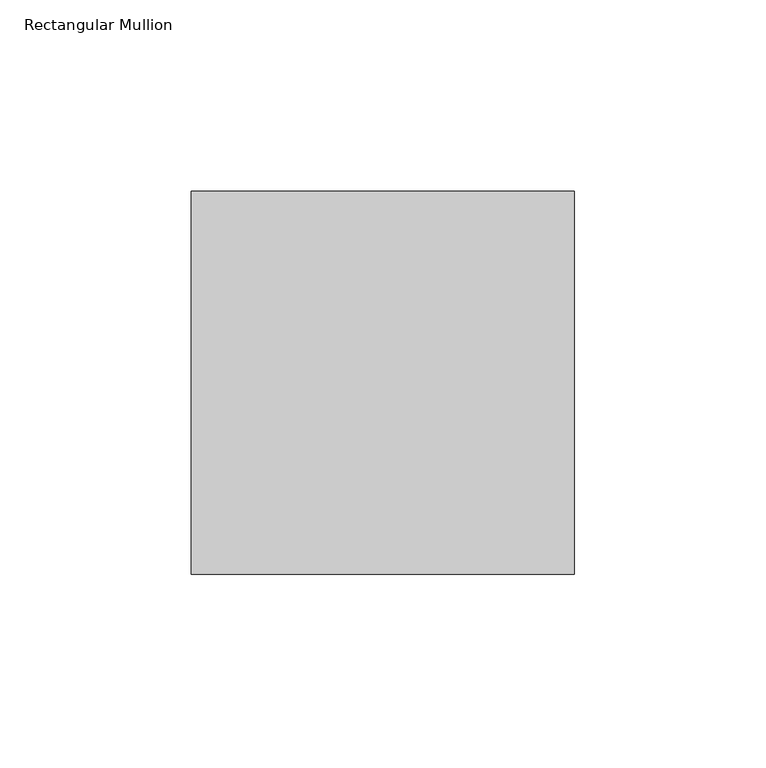
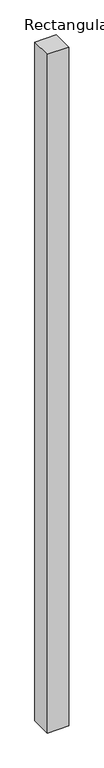
"""IFC4 building model written with IfcOpenShell, lengths in millimetres: member geometry, Rectangular Mullion : 알루미늄_Rectangular Cap_100 x100."""

import ifcopenshell
import ifcopenshell.guid

model = None  # the IFC model being written
_history = None  # IfcOwnerHistory: only IFC2X3 demands one
_inside = {}  # id of a spatial element -> (the spatial element, [elements in it])
_under = {}  # id of a project, library or spatial element -> (it, [spatial elements below it])
_declared = {}  # id of a project -> (the project, [libraries it declares])
_typed = {}  # id of a type object -> (the type object, [elements of that type])
_made_of = {}  # id of a material, layer set ... -> (it, [elements and type objects made of it])


def new_model(schema):
    """Start an empty IFC model of exactly this schema.

    Asked for "IFC4X3", IfcOpenShell would pick the latest addendum, in which some entities
    have other attributes; the version numbers below select the first issue.
    IFC2X3 requires an IfcOwnerHistory on every rooted entity: one is made here for all.
    """
    global model, _history
    if schema == "IFC4X3":
        model = ifcopenshell.file(schema_version=(4, 3, 0, 0))
    else:
        model = ifcopenshell.file(schema=schema)
    _inside.clear()
    _under.clear()
    _declared.clear()
    _typed.clear()
    _made_of.clear()
    _history = None
    if model.schema == "IFC2X3":
        org = make("IfcOrganization", Name="unknown")
        user = make(
            "IfcPersonAndOrganization",
            ThePerson=make("IfcPerson", FamilyName="unknown"),
            TheOrganization=org,
        )
        app = make(
            "IfcApplication",
            ApplicationDeveloper=org,
            Version="unknown",
            ApplicationFullName="unknown",
            ApplicationIdentifier="unknown",
        )
        _history = make(
            "IfcOwnerHistory",
            OwningUser=user,
            OwningApplication=app,
            ChangeAction="ADDED",
            CreationDate=0,
        )
    return model


def make(cls, **values):
    """One entity of the class cls with the attributes given. An attribute that is None is left unset."""
    return model.create_entity(
        cls, **{name: value for name, value in values.items() if value is not None}
    )


def rooted(cls, **values):
    """An entity with a GlobalId (a new one), such as an element, a storey or a relation."""
    return make(cls, GlobalId=ifcopenshell.guid.new(), OwnerHistory=_history, **values)


def si_unit(unit_type, name, prefix=None):
    """IfcSIUnit, for example si_unit("LENGTHUNIT", "METRE", prefix="MILLI")."""
    return make("IfcSIUnit", UnitType=unit_type, Prefix=prefix, Name=name)


def assignment(units):
    """IfcUnitAssignment: the units of a project."""
    return None if units is None else make("IfcUnitAssignment", Units=units)


def point(xyz):
    """IfcCartesianPoint."""
    return None if xyz is None else make("IfcCartesianPoint", Coordinates=xyz)


def direction(xyz):
    """IfcDirection."""
    return None if xyz is None else make("IfcDirection", DirectionRatios=xyz)


def frame(location, z_axis=None, x_axis=None):
    """IfcAxis2Placement3D, a coordinate frame: its origin and axes. An axis left out is left unset."""
    return make(
        "IfcAxis2Placement3D",
        Location=point(location),
        Axis=direction(z_axis),
        RefDirection=direction(x_axis),
    )


def origin():
    """The frame at (0, 0, 0) with its axes left unset."""
    return frame((0.0, 0.0, 0.0))


def place(relative_to, where):
    """IfcLocalPlacement: puts the frame where relative to a parent placement (None: the world)."""
    return make(
        "IfcLocalPlacement", PlacementRelTo=relative_to, RelativePlacement=where
    )


def context(
    kind, dimensions, precision=None, world=None, true_north=None, identifier=None
):
    """IfcGeometricRepresentationContext, for example the 3D "Model" context."""
    return make(
        "IfcGeometricRepresentationContext",
        ContextIdentifier=identifier,
        ContextType=kind,
        CoordinateSpaceDimension=dimensions,
        Precision=precision,
        WorldCoordinateSystem=world,
        TrueNorth=true_north,
    )


def project(units=None, contexts=None):
    """IfcProject with its units and contexts."""
    return rooted(
        "IfcProject",
        Name="project",
        RepresentationContexts=contexts,
        UnitsInContext=assignment(units),
    )


def spatial(cls, under=None, at=None, **own):
    """A site, building, storey or space (cls), placed at a placement, below another one or the project."""
    s = rooted(cls, ObjectPlacement=at, **own)
    if under is not None:
        _under.setdefault(under.id(), (under, []))[1].append(s)
    return s


def polyline(points):
    """IfcPolyline through the points."""
    return make("IfcPolyline", Points=[point(p) for p in points])


def outline(outer, holes=None, kind="AREA"):
    """IfcArbitraryClosedProfileDef: a profile drawn as a closed curve; with holes, ...WithVoids."""
    if holes is None:
        return make("IfcArbitraryClosedProfileDef", ProfileType=kind, OuterCurve=outer)
    return make(
        "IfcArbitraryProfileDefWithVoids",
        ProfileType=kind,
        OuterCurve=outer,
        InnerCurves=holes,
    )


def extrude(swept, where, along, depth):
    """IfcExtrudedAreaSolid: the profile swept, set in the frame where, extruded along a direction by depth."""
    return make(
        "IfcExtrudedAreaSolid",
        SweptArea=swept,
        Position=where,
        ExtrudedDirection=direction(along),
        Depth=depth,
    )


def shape(context_of_items, identifier, shape_type, items):
    """IfcShapeRepresentation: the items that make up one representation, for example the "Body"."""
    return make(
        "IfcShapeRepresentation",
        ContextOfItems=context_of_items,
        RepresentationIdentifier=identifier,
        RepresentationType=shape_type,
        Items=items,
    )


def source(mapping_origin, context_of_items, identifier, shape_type, items):
    """IfcRepresentationMap: a shape defined once, which mapped items show again and again."""
    return make(
        "IfcRepresentationMap",
        MappingOrigin=mapping_origin,
        MappedRepresentation=shape(context_of_items, identifier, shape_type, items),
    )


def transform(
    local_origin,
    x_axis=None,
    y_axis=None,
    z_axis=None,
    scale=None,
    scale2=None,
    scale3=None,
    uniform=True,
):
    """IfcCartesianTransformationOperator3D, or its non-uniform kind. x_axis, y_axis, z_axis: its Axis1, 2, 3."""
    if uniform:
        return make(
            "IfcCartesianTransformationOperator3D",
            Axis1=direction(x_axis),
            Axis2=direction(y_axis),
            LocalOrigin=point(local_origin),
            Scale=scale,
            Axis3=direction(z_axis),
        )
    return make(
        "IfcCartesianTransformationOperator3DnonUniform",
        Axis1=direction(x_axis),
        Axis2=direction(y_axis),
        LocalOrigin=point(local_origin),
        Scale=scale,
        Axis3=direction(z_axis),
        Scale2=scale2,
        Scale3=scale3,
    )


def mapped(mapping_source, mapping_target):
    """IfcMappedItem: shows the shape of a source again, moved by a transform."""
    return make(
        "IfcMappedItem", MappingSource=mapping_source, MappingTarget=mapping_target
    )


def made_of(thing, what):
    """Note that an element or type object is made of a material, layer set ...; save() writes the relation."""
    if what is not None:
        _made_of.setdefault(what.id(), (what, []))[1].append(thing)
    return thing


def element(
    cls,
    number,
    at=None,
    inside=None,
    cuts=None,
    type_object=None,
    material=None,
    context=None,
    identifier="Body",
    shape_type=None,
    held_by="IfcProductDefinitionShape",
    body=None,
    shapes=None,
    **own,
):
    """One element of the class cls, such as IfcWall. Its Tag is "e" and its number.

    at: its placement. inside: the storey or other place that contains it. cuts: it is an
    opening in that element (IfcRelVoidsElement). A single representation is given by context,
    identifier, shape_type and body (its items); several are given by shapes. held_by: the class
    of the entity that holds the representations. save() writes the other relations.
    """
    e = rooted(cls, Tag="e%d" % number, ObjectPlacement=at, **own)
    if body is not None:
        shapes = [shape(context, identifier, shape_type, body)]
    if shapes is not None:
        e.Representation = make(held_by, Representations=shapes)
    if inside is not None:
        _inside.setdefault(inside.id(), (inside, []))[1].append(e)
    if cuts is not None:
        rooted(
            "IfcRelVoidsElement", RelatingBuildingElement=cuts, RelatedOpeningElement=e
        )
    if type_object is not None:
        _typed.setdefault(type_object.id(), (type_object, []))[1].append(e)
    return made_of(e, material)


def aggregate(whole, parts):
    """IfcRelAggregates: a whole, such as a stair, and the parts it consists of."""
    return rooted("IfcRelAggregates", RelatingObject=whole, RelatedObjects=parts)


def save(model, path):
    """Write the relations noted so far, then the file.

    IfcRelAggregates (storeys below a building ...), IfcRelContainedInSpatialStructure (elements
    in a storey), IfcRelDefinesByType, IfcRelAssociatesMaterial and IfcRelDeclares: one each for
    every whole, place, type object, material and project.
    """
    for whole, parts in _under.values():
        aggregate(whole, parts)
    for where, things in _inside.values():
        rooted(
            "IfcRelContainedInSpatialStructure",
            RelatedElements=things,
            RelatingStructure=where,
        )
    for kind, things in _typed.values():
        rooted("IfcRelDefinesByType", RelatedObjects=things, RelatingType=kind)
    for what, things in _made_of.values():
        rooted("IfcRelAssociatesMaterial", RelatedObjects=things, RelatingMaterial=what)
    for by, libraries in _declared.values():
        rooted("IfcRelDeclares", RelatingContext=by, RelatedDefinitions=libraries)
    model.write(path)


def rectangular_mullion_9dbe7c8d(model_context):
    return source(origin(), model_context, "Body", "SweptSolid", [
        extrude(outline(polyline([(0.0, 50.0), (0.0, -50.0), (-100.0, -50.0), (-100.0, 50.0), (0.0, 50.0)])), frame((0.0, 0.0, -3325.0), z_axis=(0.0, 0.0, 1.0), x_axis=(1.0, 0.0, 0.0)), (0.0, 0.0, 1.0), 3325.0),
    ])


if __name__ == "__main__":
    model = new_model("IFC4")
    model_context = context("Model", 3, world=origin())
    ifc_project = project(units=[si_unit("LENGTHUNIT", "METRE", prefix="MILLI")], contexts=[model_context])
    site = spatial("IfcSite", under=ifc_project)
    building = spatial("IfcBuilding", under=site)
    placement = place(None, origin())
    rectangular_mullion_shape = rectangular_mullion_9dbe7c8d(model_context)
    element("IfcMember", 1, ObjectType="Rectangular Mullion : 알루미늄_Rectangular Cap_100 x100", at=placement, inside=building, context=model_context, shape_type="MappedRepresentation", body=[
        mapped(rectangular_mullion_shape, transform((0.0, 0.0, 0.0), x_axis=(1.0, 0.0, 0.0), y_axis=(0.0, 1.0, 0.0), z_axis=(0.0, 0.0, 1.0))),
    ])
    save(model, "model.ifc")

# Revit data of these elements
# Type "Rectangular Mullion : 알루미늄_Rectangular Cap_100 x100"
#   built-in parameter 1007304 = 0.328084 (stored number, unit not read)
#   built-in parameter 1007301 = 0.164042 (stored number, unit not read)
#   built-in parameter 1007300 = 0.164042 (stored number, unit not read)
# Element 1 (IfcMember, "Rectangular Mullion : 알루미늄_Rectangular Cap_100 x100")
#   Materials on its faces: "00_Metal_Stainless Steel"
# Materials
#   "00_Metal_Stainless Steel": class "Metal", colour RGB 148 148 148, transparency 0, Description = "Steel", Cost = 0
